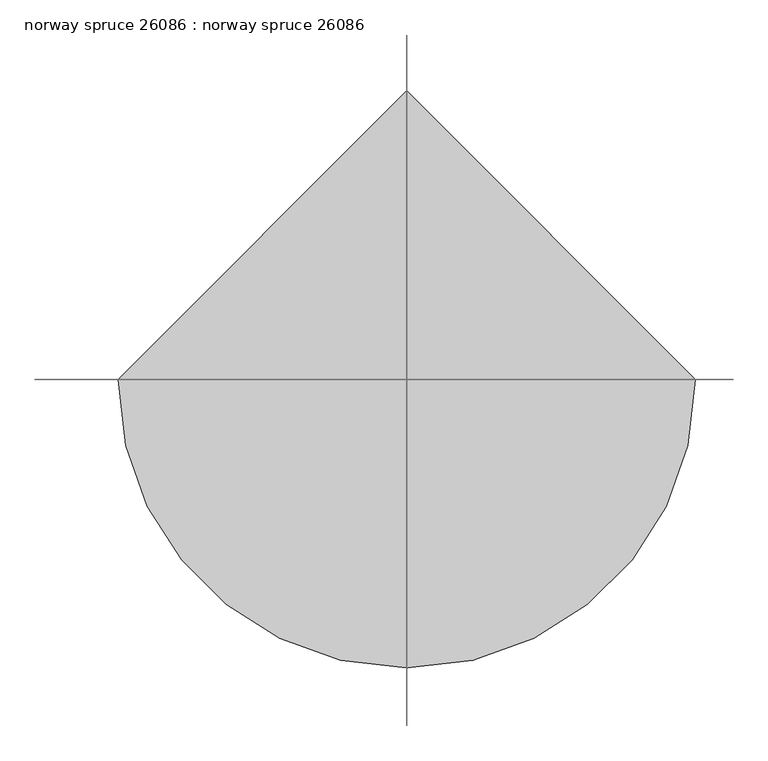
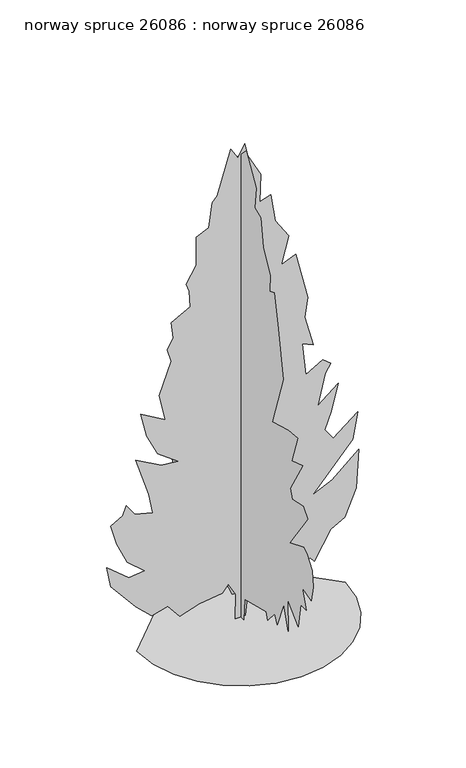
"""IFC4 building model written with IfcOpenShell, lengths in millimetres: proxy geometry, norway spruce 26086 : norway spruce 26086."""

from ifc_helpers import new_model, si_unit, origin, place, context, project, spatial, triangles, source, transform, mapped, element, save


def norway_spruce_26086_norway_spruce_26086_64d82020(model_context):
    return source(origin(), model_context, "Body", "Tessellation", [
        triangles([(-954.9721601, 0.0, 2.42e-05), (-929.7245733, -218.8163494, 2.42e-05), (-857.8247469, -419.7632589, 2.42e-05), (-745.0257454, -597.0859019, 2.42e-05), (-597.0859019, -745.0257454, 2.42e-05), (-419.7632589, -857.8247469, 2.42e-05), (-218.816095, -929.7245733, 2.42e-05), (4.17e-05, -954.9721601, 2.42e-05), (218.8163494, -929.7245733, 2.42e-05), (419.7632589, -857.8247469, 2.42e-05), (597.0859019, -745.0257454, 2.42e-05), (745.0257454, -597.0859019, 2.42e-05), (857.8247469, -419.7632589, 2.42e-05), (929.7245733, -218.816095, 2.42e-05), (954.9721601, 8.35e-05, 2.42e-05), (-0.0001252, 954.9721601, 2.42e-05), (-52.0131451, 2.3e-06, 4.1e-06), (-45.7469624, -1.19e-05, 233.9905685), (-114.4303972, -1.64e-05, 358.8946632), (-169.0439877, -9.8e-06, 288.6763112), (-379.1994558, 1.2e-06, 258.1937423), (-559.1458849, 1.24e-05, 202.8534611), (-668.3761362, 9.2e-06, 335.4885338), (-816.615707, 1.8e-05, 296.4791961), (-964.852807, 1.61e-05, 436.9159184), (-1191.113633, 9.7e-06, 709.9864597), (-1230.1230251, -2e-07, 905.0382895), (-1027.2707994, 7e-07, 741.1954559), (-879.0312286, -6.7e-06, 756.7987186), (-1042.8740622, -7.9e-06, 897.2354227), (-1136.4985073, -1.59e-05, 1100.0901192), (-1191.113633, -2.51e-05, 1295.1420216), (-1081.8833817, -3.36e-05, 1357.5573978), (-1050.6769289, -4.01e-05, 1443.3790489), (-972.6556738, -3.7e-05, 1334.1512684), (-808.8128403, -4.18e-05, 1295.1420216), (-842.6787237, -5.17e-05, 1484.6641743), (-964.852807, -6.85e-05, 1856.8888378), (-730.7915852, -7.08e-05, 1724.252457), (-574.2893646, -7.68e-05, 1709.7591557), (-762.0005814, -7.69e-05, 1849.0859711), (-863.4279659, -8.46e-05, 2051.9405949), (-918.0405481, -9.61e-05, 2286.0018894), (-691.7822657, -9.81e-05, 2153.3655087), (-746.3948479, -0.0001106, 2403.0323914), (-637.16714, -0.0001331, 2699.5142944), (-676.1764595, -0.0001388, 2824.3552208), (-621.5638773, -0.0001472, 2925.7775185), (-637.16714, -0.0001554, 3074.012075), (-465.5214034, -0.0001685, 3167.6365929), (-473.7865966, -0.0001773, 3322.3989487), (-501.9145672, -0.0001809, 3402.2818634), (-410.9062778, -0.0001936, 3549.9321533), (-410.9062778, -0.0002099, 3823.0079269), (-295.541935, -0.000218, 3874.3158417), (-262.6692322, -0.0002331, 4103.8811897), (-215.8559741, -0.0002384, 4158.4912285), (-91.0235138, -0.0002681, 4564.2057083), (-28.607027, -0.0002648, 4462.7837013), (33.8094597, -0.000274, 4572.0037788), (65.0179563, -0.0002679, 4447.1625618), (182.0485537, -0.00026, 4228.7224068), (174.2464318, -0.0002439, 3963.4447037), (275.6715091, -0.0002501, 3994.6611122), (314.6834084, -0.000236, 3729.3834091), (439.516886, -0.0002303, 3542.1343735), (369.2984977, -0.0002119, 3284.6544502), (501.932335, -0.000221, 3339.2897781), (611.1626226, -0.0001988, 2886.7630394), (587.7564569, -0.0001866, 2699.5142944), (665.7752048, -0.0001723, 2403.0323914), (564.3503637, -0.0001707, 2449.8446503), (595.5568165, -0.0001535, 2137.7622459), (751.5993267, -0.0001659, 2231.3867638), (821.8176424, -0.0001652, 2168.9712421), (775.0054562, -0.0001585, 2090.949987), (704.7870678, -0.0001382, 1802.2737122), (892.0360308, -0.0001553, 1950.5132103), (829.6180384, -0.0001376, 1700.8487984), (767.2025167, -0.0001256, 1544.8064335), (845.2237719, -0.0001225, 1435.578653), (1071.4820543, -0.0001431, 1615.0246765), (1024.6698681, -0.0001262, 1365.3602646), (657.9748089, -8.55e-05, 951.8505484), (837.4209051, -9.85e-05, 1037.6721268), (1079.3611519, -0.0001214, 1245.4696175), (1055.8788643, -9.87e-05, 881.63216), (954.4514797, -7.94e-05, 631.9652046), (821.8176424, -6.94e-05, 561.7468526), (673.5780716, -4.76e-05, 304.2795376), (634.5686794, -4.87e-05, 351.0917965), (369.2984977, -2.4e-05, 132.6348456), (345.8924046, -2.91e-05, 234.0616942), (135.2360586, -1.47e-05, 148.2390894), (65.017702, -1.54e-05, 210.6553286), (41.6113273, -1.8e-06, 0.0), (2.1e-06, 47.3113473, 2.84e-05), (8.7e-06, 70.7174676, 187.2491992), (1.01e-05, 133.1339521, 140.4369675), (1.64e-05, 242.3629317, 187.2491992), (2.32e-05, 382.7986184, 202.8534611), (3.05e-05, 546.6439954, 202.8534611), (3.7e-05, 587.3043406, 362.1915914), (4.1e-05, 710.7459337, 309.7887943), (4.73e-05, 772.9023142, 429.1130153), (6.07e-05, 952.3508812, 608.5590752), (7.81e-05, 1123.9941107, 936.2472857), (8.19e-05, 1139.5998442, 1037.6721268), (6.4e-05, 811.9116337, 928.4444189), (7.9e-05, 1006.9634634, 1139.0994387), (9.36e-05, 1119.7776529, 1460.6409313), (8.24e-05, 908.7847904, 1401.7661819), (8.72e-05, 905.5361515, 1568.2125629), (8.01e-05, 772.9023142, 1529.2031708), (8.81e-05, 827.5174398, 1716.4520611), (9.88e-05, 843.1206299, 2051.9405949), (8.05e-05, 515.4349992, 1927.1072262), (9.28e-05, 640.2684769, 2153.3679794), (0.0001013, 601.2565776, 2496.6569092), (0.0001109, 671.4749296, 2715.1098541), (0.0001132, 567.9546132, 2944.9036766), (0.0001197, 559.9028154, 3177.6441216), (0.0001155, 398.4043882, 3276.8566704), (0.0001214, 437.4137441, 3417.2934471), (0.0001235, 308.7626578, 3682.0124634), (0.0001285, 273.5709105, 3901.0365944), (0.0001262, 211.1544261, 3916.6324448), (0.0001321, 94.123588, 4291.1302254), (0.0001344, 62.9153412, 4415.9714424), (0.0001324, -85.3229897, 4572.0037788), (0.0001173, -241.3647005, 4298.9280052), (0.0001123, -217.9585892, 4096.0834099), (0.0001069, -319.3849382, 4064.8667107), (9.72e-05, -358.3968375, 3799.5890076), (8.63e-05, -467.6245454, 3596.7444122), (8.18e-05, -459.8216423, 3432.914296), (7.95e-05, -530.0399943, 3464.105706), (6.75e-05, -592.4580231, 3152.0410332), (5.07e-05, -670.4767347, 2707.3120743), (4.3e-05, -498.8335416, 2192.3773716), (3.4e-05, -749.4961847, 2265.5522655), (2.75e-05, -904.5378839, 2278.1988773), (2.35e-05, -810.9134388, 2005.128336), (1.75e-05, -982.5591391, 2059.7409908), (1.62e-05, -787.5073093, 1724.2549278), (1.22e-05, -818.7163055, 1638.430806), (5.5e-06, -992.5565666, 1672.3220512), (0.0, -1060.5803942, 1591.6185471), (7e-07, -779.706986, 1193.7145643), (-6.5e-06, -998.1649452, 1279.5361427), (-1.01e-05, -1052.7775274, 1240.5268959), (-1.68e-05, -1130.7987099, 1131.2965719), (-2.2e-05, -1146.4019726, 983.0595446), (-2.5e-05, -1115.1955198, 834.8199011), (-1.75e-05, -974.7588158, 873.8292933), (-2.57e-05, -1037.1742647, 694.383197), (-2.18e-05, -951.3526863, 694.383197), (-2.71e-05, -912.3408234, 460.3220115), (-1.47e-05, -740.6950504, 616.3619419), (-2.43e-05, -756.3008566, 319.8853074), (-1.45e-05, -678.2796015, 530.5403998), (-1.76e-05, -576.8522532, 273.0730848), (-1.33e-05, -537.8428974, 358.8946632), (-1.24e-05, -428.6126461, 226.2595724), (-9.3e-06, -405.2065166, 296.4791961), (3.5e-06, -61.9173734, 210.655583), (-2.1e-06, -46.3131251, 2.56e-05)], [[15, 16, 1], [14, 15, 1], [14, 1, 2], [13, 14, 2], [13, 2, 3], [13, 3, 4], [12, 13, 4], [11, 12, 4], [11, 4, 5], [11, 5, 6], [11, 6, 7], [11, 7, 8], [11, 8, 9], [11, 9, 10], [77, 78, 79], [81, 82, 83], [37, 38, 39], [59, 60, 61], [85, 86, 87], [42, 43, 44], [57, 58, 59], [70, 71, 72], [33, 34, 35], [91, 92, 93], [89, 90, 91], [81, 83, 84], [26, 27, 28], [25, 26, 28], [67, 68, 69], [63, 64, 65], [25, 28, 29], [96, 17, 18], [95, 96, 18], [41, 42, 44], [74, 75, 76], [73, 74, 76], [73, 76, 77], [85, 87, 88], [84, 85, 88], [84, 88, 89], [31, 32, 33], [31, 33, 35], [77, 79, 80], [37, 39, 40], [31, 35, 36], [30, 31, 36], [29, 30, 36], [21, 22, 23], [48, 49, 50], [40, 41, 44], [53, 54, 55], [84, 89, 91], [84, 91, 93], [93, 94, 95], [84, 93, 95], [84, 95, 18], [84, 18, 19], [24, 25, 29], [23, 24, 29], [36, 37, 40], [80, 81, 84], [59, 61, 62], [57, 59, 62], [57, 62, 63], [56, 57, 63], [55, 56, 63], [55, 63, 65], [53, 55, 65], [53, 65, 66], [53, 66, 67], [52, 53, 67], [51, 52, 67], [50, 51, 67], [50, 67, 69], [50, 69, 70], [48, 50, 70], [48, 70, 72], [47, 48, 72], [46, 47, 72], [45, 46, 72], [44, 45, 72], [44, 72, 73], [40, 44, 73], [40, 73, 77], [40, 77, 80], [40, 80, 84], [40, 84, 19], [36, 40, 19], [29, 36, 19], [23, 29, 19], [21, 23, 19], [20, 21, 19], [159, 160, 161], [143, 144, 145], [161, 162, 163], [110, 111, 112], [157, 158, 159], [163, 164, 165], [107, 108, 109], [106, 107, 109], [141, 142, 143], [115, 116, 117], [155, 156, 157], [129, 130, 131], [112, 113, 114], [136, 137, 138], [128, 129, 131], [128, 131, 132], [127, 128, 132], [153, 154, 155], [140, 141, 143], [166, 167, 97], [166, 97, 98], [103, 104, 105], [101, 102, 103], [147, 148, 149], [146, 147, 149], [114, 115, 117], [105, 106, 109], [125, 126, 127], [103, 105, 109], [132, 133, 134], [127, 132, 134], [125, 127, 134], [125, 134, 135], [125, 135, 136], [124, 125, 136], [123, 124, 136], [123, 136, 138], [123, 138, 139], [123, 139, 140], [122, 123, 140], [121, 122, 140], [120, 121, 140], [119, 120, 140], [118, 119, 140], [117, 118, 140], [140, 143, 145], [117, 140, 145], [114, 117, 145], [114, 145, 146], [114, 146, 149], [152, 153, 155], [151, 152, 155], [150, 151, 155], [149, 150, 155], [109, 110, 112], [155, 157, 159], [149, 155, 159], [114, 149, 159], [114, 159, 161], [114, 161, 163], [114, 163, 165], [114, 165, 166], [114, 166, 98], [112, 114, 98], [109, 112, 98], [103, 109, 98], [101, 103, 98], [100, 101, 98], [99, 100, 98]], closed=False),
    ])


if __name__ == "__main__":
    model = new_model("IFC4")
    model_context = context("Model", 3, world=origin())
    ifc_project = project(units=[si_unit("LENGTHUNIT", "METRE", prefix="MILLI")], contexts=[model_context])
    site = spatial("IfcSite", under=ifc_project)
    building = spatial("IfcBuilding", under=site)
    placement = place(None, origin())
    norway_spruce_26086_norway_spruce_26086_shape = norway_spruce_26086_norway_spruce_26086_64d82020(model_context)
    element("IfcBuildingElementProxy", 1, Name="norway spruce 26086 : norway spruce 26086", ObjectType="norway spruce 26086 : norway spruce 26086", at=placement, inside=building, context=model_context, shape_type="MappedRepresentation", body=[
        mapped(norway_spruce_26086_norway_spruce_26086_shape, transform((0.0, 0.0, 0.0), x_axis=(1.0, 0.0, 0.0), y_axis=(0.0, 1.0, 0.0), z_axis=(0.0, 0.0, 1.0))),
    ])
    save(model, "model.ifc")

# Revit data of these elements
# Type "norway spruce 26086 : norway spruce 26086"
#   built-in parameter 1005195 = "RPC-16-FXGW-0XFX-PJ97-W000-ST1L-LVER-AU"
#   Height = 0
